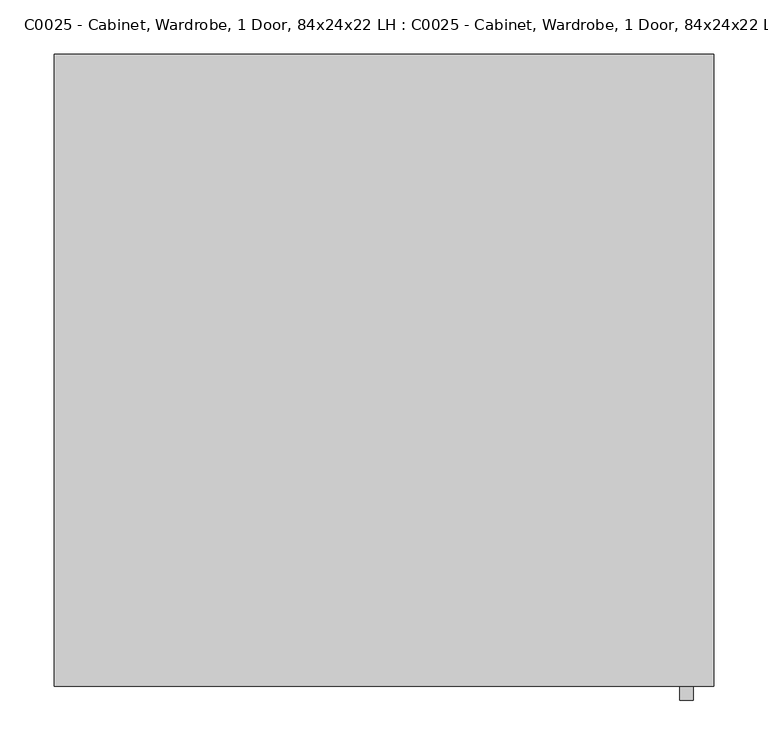
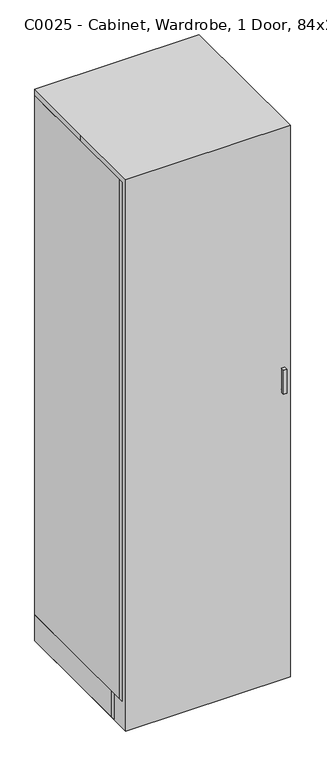
"""IFC4 building model written with IfcOpenShell, lengths in millimetres: proxy geometry, C0025 - Cabinet, Wardrobe, 1 Door, 84x24x22 LH : C0025 - Cabinet, Wardrobe, 1 Door, 84x24x22 LH."""

import ifcopenshell
import ifcopenshell.guid

model = None  # the IFC model being written
_history = None  # IfcOwnerHistory: only IFC2X3 demands one
_inside = {}  # id of a spatial element -> (the spatial element, [elements in it])
_under = {}  # id of a project, library or spatial element -> (it, [spatial elements below it])
_declared = {}  # id of a project -> (the project, [libraries it declares])
_typed = {}  # id of a type object -> (the type object, [elements of that type])
_made_of = {}  # id of a material, layer set ... -> (it, [elements and type objects made of it])


def new_model(schema):
    """Start an empty IFC model of exactly this schema.

    Asked for "IFC4X3", IfcOpenShell would pick the latest addendum, in which some entities
    have other attributes; the version numbers below select the first issue.
    IFC2X3 requires an IfcOwnerHistory on every rooted entity: one is made here for all.
    """
    global model, _history
    if schema == "IFC4X3":
        model = ifcopenshell.file(schema_version=(4, 3, 0, 0))
    else:
        model = ifcopenshell.file(schema=schema)
    _inside.clear()
    _under.clear()
    _declared.clear()
    _typed.clear()
    _made_of.clear()
    _history = None
    if model.schema == "IFC2X3":
        org = make("IfcOrganization", Name="unknown")
        user = make(
            "IfcPersonAndOrganization",
            ThePerson=make("IfcPerson", FamilyName="unknown"),
            TheOrganization=org,
        )
        app = make(
            "IfcApplication",
            ApplicationDeveloper=org,
            Version="unknown",
            ApplicationFullName="unknown",
            ApplicationIdentifier="unknown",
        )
        _history = make(
            "IfcOwnerHistory",
            OwningUser=user,
            OwningApplication=app,
            ChangeAction="ADDED",
            CreationDate=0,
        )
    return model


def make(cls, **values):
    """One entity of the class cls with the attributes given. An attribute that is None is left unset."""
    return model.create_entity(
        cls, **{name: value for name, value in values.items() if value is not None}
    )


def rooted(cls, **values):
    """An entity with a GlobalId (a new one), such as an element, a storey or a relation."""
    return make(cls, GlobalId=ifcopenshell.guid.new(), OwnerHistory=_history, **values)


def si_unit(unit_type, name, prefix=None):
    """IfcSIUnit, for example si_unit("LENGTHUNIT", "METRE", prefix="MILLI")."""
    return make("IfcSIUnit", UnitType=unit_type, Prefix=prefix, Name=name)


def assignment(units):
    """IfcUnitAssignment: the units of a project."""
    return None if units is None else make("IfcUnitAssignment", Units=units)


def point(xyz):
    """IfcCartesianPoint."""
    return None if xyz is None else make("IfcCartesianPoint", Coordinates=xyz)


def direction(xyz):
    """IfcDirection."""
    return None if xyz is None else make("IfcDirection", DirectionRatios=xyz)


def frame(location, z_axis=None, x_axis=None):
    """IfcAxis2Placement3D, a coordinate frame: its origin and axes. An axis left out is left unset."""
    return make(
        "IfcAxis2Placement3D",
        Location=point(location),
        Axis=direction(z_axis),
        RefDirection=direction(x_axis),
    )


def frame_2d(location, x_axis=None):
    """IfcAxis2Placement2D, a coordinate frame in the plane: its origin and x axis."""
    return make(
        "IfcAxis2Placement2D", Location=point(location), RefDirection=direction(x_axis)
    )


def origin():
    """The frame at (0, 0, 0) with its axes left unset."""
    return frame((0.0, 0.0, 0.0))


def origin_with_axes():
    """The frame at (0, 0, 0) with the z axis (0, 0, 1) and the x axis (1, 0, 0) written out."""
    return frame((0.0, 0.0, 0.0), z_axis=(0.0, 0.0, 1.0), x_axis=(1.0, 0.0, 0.0))


def place(relative_to, where):
    """IfcLocalPlacement: puts the frame where relative to a parent placement (None: the world)."""
    return make(
        "IfcLocalPlacement", PlacementRelTo=relative_to, RelativePlacement=where
    )


def context(
    kind, dimensions, precision=None, world=None, true_north=None, identifier=None
):
    """IfcGeometricRepresentationContext, for example the 3D "Model" context."""
    return make(
        "IfcGeometricRepresentationContext",
        ContextIdentifier=identifier,
        ContextType=kind,
        CoordinateSpaceDimension=dimensions,
        Precision=precision,
        WorldCoordinateSystem=world,
        TrueNorth=true_north,
    )


def project(units=None, contexts=None):
    """IfcProject with its units and contexts."""
    return rooted(
        "IfcProject",
        Name="project",
        RepresentationContexts=contexts,
        UnitsInContext=assignment(units),
    )


def spatial(cls, under=None, at=None, **own):
    """A site, building, storey or space (cls), placed at a placement, below another one or the project."""
    s = rooted(cls, ObjectPlacement=at, **own)
    if under is not None:
        _under.setdefault(under.id(), (under, []))[1].append(s)
    return s


def polyline(points):
    """IfcPolyline through the points."""
    return make("IfcPolyline", Points=[point(p) for p in points])


def circle_curve(where, radius):
    """IfcCircle in the frame where."""
    return make("IfcCircle", Position=where, Radius=radius)


def trimmed(basis, trim1, trim2, sense, master):
    """IfcTrimmedCurve: the piece of a basis curve between two trims."""
    return make(
        "IfcTrimmedCurve",
        BasisCurve=basis,
        Trim1=trim1,
        Trim2=trim2,
        SenseAgreement=sense,
        MasterRepresentation=master,
    )


def segment(curve, same_sense, transition):
    """IfcCompositeCurveSegment."""
    return make(
        "IfcCompositeCurveSegment",
        Transition=transition,
        SameSense=same_sense,
        ParentCurve=curve,
    )


def composite_curve(segments, self_intersect=None):
    """IfcCompositeCurve: segments joined end to end."""
    return make("IfcCompositeCurve", Segments=segments, SelfIntersect=self_intersect)


def outline(outer, holes=None, kind="AREA"):
    """IfcArbitraryClosedProfileDef: a profile drawn as a closed curve; with holes, ...WithVoids."""
    if holes is None:
        return make("IfcArbitraryClosedProfileDef", ProfileType=kind, OuterCurve=outer)
    return make(
        "IfcArbitraryProfileDefWithVoids",
        ProfileType=kind,
        OuterCurve=outer,
        InnerCurves=holes,
    )


def extrude(swept, where, along, depth):
    """IfcExtrudedAreaSolid: the profile swept, set in the frame where, extruded along a direction by depth."""
    return make(
        "IfcExtrudedAreaSolid",
        SweptArea=swept,
        Position=where,
        ExtrudedDirection=direction(along),
        Depth=depth,
    )


def shape(context_of_items, identifier, shape_type, items):
    """IfcShapeRepresentation: the items that make up one representation, for example the "Body"."""
    return make(
        "IfcShapeRepresentation",
        ContextOfItems=context_of_items,
        RepresentationIdentifier=identifier,
        RepresentationType=shape_type,
        Items=items,
    )


def source(mapping_origin, context_of_items, identifier, shape_type, items):
    """IfcRepresentationMap: a shape defined once, which mapped items show again and again."""
    return make(
        "IfcRepresentationMap",
        MappingOrigin=mapping_origin,
        MappedRepresentation=shape(context_of_items, identifier, shape_type, items),
    )


def transform(
    local_origin,
    x_axis=None,
    y_axis=None,
    z_axis=None,
    scale=None,
    scale2=None,
    scale3=None,
    uniform=True,
):
    """IfcCartesianTransformationOperator3D, or its non-uniform kind. x_axis, y_axis, z_axis: its Axis1, 2, 3."""
    if uniform:
        return make(
            "IfcCartesianTransformationOperator3D",
            Axis1=direction(x_axis),
            Axis2=direction(y_axis),
            LocalOrigin=point(local_origin),
            Scale=scale,
            Axis3=direction(z_axis),
        )
    return make(
        "IfcCartesianTransformationOperator3DnonUniform",
        Axis1=direction(x_axis),
        Axis2=direction(y_axis),
        LocalOrigin=point(local_origin),
        Scale=scale,
        Axis3=direction(z_axis),
        Scale2=scale2,
        Scale3=scale3,
    )


def mapped(mapping_source, mapping_target):
    """IfcMappedItem: shows the shape of a source again, moved by a transform."""
    return make(
        "IfcMappedItem", MappingSource=mapping_source, MappingTarget=mapping_target
    )


def made_of(thing, what):
    """Note that an element or type object is made of a material, layer set ...; save() writes the relation."""
    if what is not None:
        _made_of.setdefault(what.id(), (what, []))[1].append(thing)
    return thing


def element(
    cls,
    number,
    at=None,
    inside=None,
    cuts=None,
    type_object=None,
    material=None,
    context=None,
    identifier="Body",
    shape_type=None,
    held_by="IfcProductDefinitionShape",
    body=None,
    shapes=None,
    **own,
):
    """One element of the class cls, such as IfcWall. Its Tag is "e" and its number.

    at: its placement. inside: the storey or other place that contains it. cuts: it is an
    opening in that element (IfcRelVoidsElement). A single representation is given by context,
    identifier, shape_type and body (its items); several are given by shapes. held_by: the class
    of the entity that holds the representations. save() writes the other relations.
    """
    e = rooted(cls, Tag="e%d" % number, ObjectPlacement=at, **own)
    if body is not None:
        shapes = [shape(context, identifier, shape_type, body)]
    if shapes is not None:
        e.Representation = make(held_by, Representations=shapes)
    if inside is not None:
        _inside.setdefault(inside.id(), (inside, []))[1].append(e)
    if cuts is not None:
        rooted(
            "IfcRelVoidsElement", RelatingBuildingElement=cuts, RelatedOpeningElement=e
        )
    if type_object is not None:
        _typed.setdefault(type_object.id(), (type_object, []))[1].append(e)
    return made_of(e, material)


def aggregate(whole, parts):
    """IfcRelAggregates: a whole, such as a stair, and the parts it consists of."""
    return rooted("IfcRelAggregates", RelatingObject=whole, RelatedObjects=parts)


def save(model, path):
    """Write the relations noted so far, then the file.

    IfcRelAggregates (storeys below a building ...), IfcRelContainedInSpatialStructure (elements
    in a storey), IfcRelDefinesByType, IfcRelAssociatesMaterial and IfcRelDeclares: one each for
    every whole, place, type object, material and project.
    """
    for whole, parts in _under.values():
        aggregate(whole, parts)
    for where, things in _inside.values():
        rooted(
            "IfcRelContainedInSpatialStructure",
            RelatedElements=things,
            RelatingStructure=where,
        )
    for kind, things in _typed.values():
        rooted("IfcRelDefinesByType", RelatedObjects=things, RelatingType=kind)
    for what, things in _made_of.values():
        rooted("IfcRelAssociatesMaterial", RelatedObjects=things, RelatingMaterial=what)
    for by, libraries in _declared.values():
        rooted("IfcRelDeclares", RelatingContext=by, RelatedDefinitions=libraries)
    model.write(path)


def c0025_cabinet_wardrobe_1_door_84x24x22_lh_c0025_cabinet_367b7b03(model_context):
    return source(origin(), model_context, "Body", "SweptSolid", [
        extrude(outline(polyline([(-304.7810937, 1219.2), (-266.7, 1219.2), (-266.7, 1206.5303499), (-292.1114436, 1206.5303499), (-292.1114436, 1136.6574627), (-266.7, 1136.6574627), (-266.7, 1123.9878126), (-304.7810937, 1123.9878126), (-304.7810937, 1219.2)])), frame((273.1988281, 0.0, 0.0), z_axis=(1.0, 0.0, 0.0), x_axis=(0.0, 1.0, 0.0)), (0.0, 0.0, 1.0), 12.4023437),
        extrude(outline(polyline([(-304.8, -247.65), (-304.8, 292.1), (-285.75, 292.1), (-285.75, -247.65), (-304.8, -247.65)])), frame((0.0, 0.0, 101.6), z_axis=(0.0, 0.0, 1.0), x_axis=(1.0, 0.0, 0.0)), (0.0, 0.0, 1.0), 2032.0),
        extrude(outline(polyline([(304.8, 292.1), (304.8, -247.65), (285.75, -247.65), (285.75, 292.1), (304.8, 292.1)])), frame((0.0, 0.0, 101.6), z_axis=(0.0, 0.0, 1.0), x_axis=(1.0, 0.0, 0.0)), (0.0, 0.0, 1.0), 2032.0),
        extrude(outline(composite_curve([segment(trimmed(circle_curve(frame_2d((0.0, 1572.32055)), 12.7), [point((-12.7, 1572.32055))], [point((12.7, 1572.32055))], False, "CARTESIAN"), True, "CONTINUOUS"), segment(trimmed(circle_curve(frame_2d((0.0, 1572.32055)), 12.7), [point((12.7, 1572.32055))], [point((-12.7, 1572.32055))], False, "CARTESIAN"), True, "CONTINUOUS")], self_intersect=False)), frame((-285.75, 0.0, 0.0), z_axis=(1.0, 0.0, 0.0), x_axis=(0.0, 1.0, 0.0)), (0.0, 0.0, 1.0), 571.5),
        extrude(outline(polyline([(285.75, -247.65), (-285.75, -247.65), (-285.75, 273.05), (285.75, 273.05), (285.75, -247.65)])), frame((0.0, 0.0, 1689.1), z_axis=(0.0, 0.0, 1.0), x_axis=(1.0, 0.0, 0.0)), (0.0, 0.0, 1.0), 25.4),
        extrude(outline(polyline([(285.75, 292.1), (285.75, -247.65), (-285.75, -247.65), (-285.75, 292.1), (285.75, 292.1)])), frame((0.0, 0.0, 2114.55), z_axis=(0.0, 0.0, 1.0), x_axis=(1.0, 0.0, 0.0)), (0.0, 0.0, 1.0), 19.05),
        extrude(outline(polyline([(304.8, -266.7), (-304.8, -266.7), (-304.8, -247.65), (304.8, -247.65), (304.8, -266.7)])), frame((0.0, 0.0, 101.6), z_axis=(0.0, 0.0, 1.0), x_axis=(1.0, 0.0, 0.0)), (0.0, 0.0, 1.0), 2032.0),
        extrude(outline(polyline([(285.75, 273.05), (-285.75, 273.05), (-285.75, 292.1), (285.75, 292.1), (285.75, 273.05)])), origin_with_axes(), (0.0, 0.0, 1.0), 2114.55),
        extrude(outline(polyline([(-285.75, 292.1), (-285.75, -196.85), (-304.8, -196.85), (-304.8, 292.1), (-285.75, 292.1)])), origin_with_axes(), (0.0, 0.0, 1.0), 101.6),
        extrude(outline(polyline([(304.8, 292.1), (304.8, -196.85), (285.75, -196.85), (285.75, 292.1), (304.8, 292.1)])), origin_with_axes(), (0.0, 0.0, 1.0), 101.6),
        extrude(outline(polyline([(285.75, -247.65), (-285.75, -247.65), (-285.75, 273.05), (285.75, 273.05), (285.75, -247.65)])), frame((0.0, 0.0, 101.6), z_axis=(0.0, 0.0, 1.0), x_axis=(1.0, 0.0, 0.0)), (0.0, 0.0, 1.0), 25.4),
        extrude(outline(polyline([(304.8, -196.85), (304.8, -215.9), (-304.8, -215.9), (-304.8, -196.85), (304.8, -196.85)])), origin_with_axes(), (0.0, 0.0, 1.0), 101.6),
        extrude(outline(polyline([(-304.8, 292.1), (304.8, 292.1), (304.8, -292.1), (-304.8, -292.1), (-304.8, 0.0), (-304.8, 292.1)])), origin_with_axes(), (0.0, 0.0, 1.0), 2159.0),
    ])


if __name__ == "__main__":
    model = new_model("IFC4")
    model_context = context("Model", 3, world=origin())
    ifc_project = project(units=[si_unit("LENGTHUNIT", "METRE", prefix="MILLI")], contexts=[model_context])
    site = spatial("IfcSite", under=ifc_project)
    building = spatial("IfcBuilding", under=site)
    placement = place(None, origin())
    c0025_cabinet_wardrobe_1_door_84x24x22_lh_c0025_cabinet_shape = c0025_cabinet_wardrobe_1_door_84x24x22_lh_c0025_cabinet_367b7b03(model_context)
    element("IfcBuildingElementProxy", 1, Name="C0025 - Cabinet, Wardrobe, 1 Door, 84x24x22 LH : C0025 - Cabinet, Wardrobe, 1 Door, 84x24x22 LH", ObjectType="C0025 - Cabinet, Wardrobe, 1 Door, 84x24x22 LH : C0025 - Cabinet, Wardrobe, 1 Door, 84x24x22 LH", at=placement, inside=building, context=model_context, shape_type="MappedRepresentation", body=[
        mapped(c0025_cabinet_wardrobe_1_door_84x24x22_lh_c0025_cabinet_shape, transform((0.0, 0.0, 0.0), x_axis=(1.0, 0.0, 0.0), y_axis=(0.0, 1.0, 0.0), z_axis=(0.0, 0.0, 1.0))),
    ])
    save(model, "model.ifc")

# Revit data of these elements
# Type "C0025 - Cabinet, Wardrobe, 1 Door, 84x24x22 LH : C0025 - Cabinet, Wardrobe, 1 Door, 84x24x22 LH"
#   Watts2 = "0"
#   Watts1 = "0"
#   Unit_Issue = "EA"
#   UTIL_6_Misc = "-"
#   UTIL_5_NonMedGas = "-"
#   UTIL_4_MiscGas = "-"
#   UTIL_3_MedGas = "-"
#   UTIL_2_Elec = "-"
#   UTIL_1_WaterDrain = "-"
#   Nomenclature = "Cabinet, Wardrobe, 1 Door, 84x24x22"
#   NSN = "6530"
#   Location [instance default] = ""
#   JSN = "C0025"
#   Fund_Source_VA = "-"
#   Fund_Source_Navy = "-"
#   Fund_Source_Army = "-"
#   Fund_Source_AF = "-"
#   ELEC_Volts2 = "0"
#   ELEC_Volts1 = "0"
#   ELEC_Phase2 = "0"
#   ELEC_Phase1 = "0"
#   ELEC_HertzSwitch = "0"
#   ELEC_HertzDependent = "0"
#   ELEC_Hertz = "0"
#   ELEC_Amps2 = "0"
#   ELEC_Amps1 = "0"
#   DetailDescription = "Wardrobe cabinet with a fixed shelf, clothing rod, and a solid or louvered right or left-hinged door (appropriate door hinge configuration to be indicated on the equipment elevation drawings), an optional locking door is available. Also referred to as a wardrobe case, unit or storage unit. Used for storage of clothing and personal items."
#   CAT_VA = "A"
#   CAT_Navy = "A"
#   CAT_IHS = "-"
#   CAT_Army = "A"
#   CAT_AF = "A"
#   BTUperhour = "0"
#   Weight_IP = 219
#   DIM_Width_IP = 2' - 0"
#   DIM_Height_IP = 7' - 1"
#   DIM_Depth_IP = 1' - 11"
# Element 1 (IfcBuildingElementProxy, "C0025 - Cabinet, Wardrobe, 1 Door, 84x24x22 LH : C0025 - Cabinet, Wardrobe, 1 Door, 84x24x22 LH")
#   Location = "DUTY1"
#   Materials on its faces: "CabinetFinish", "Default metal", "EquipSpace"
# Materials
#   "CabinetFinish": class "Unassigned", colour RGB 245 239 218, transparency 0
#   "Default metal": class "Unassigned", colour RGB 204 204 204, transparency 0
#   "EquipSpace": class "Unassigned", colour RGB 221 217 195, transparency 0.5
